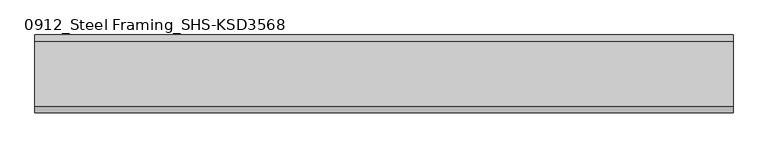
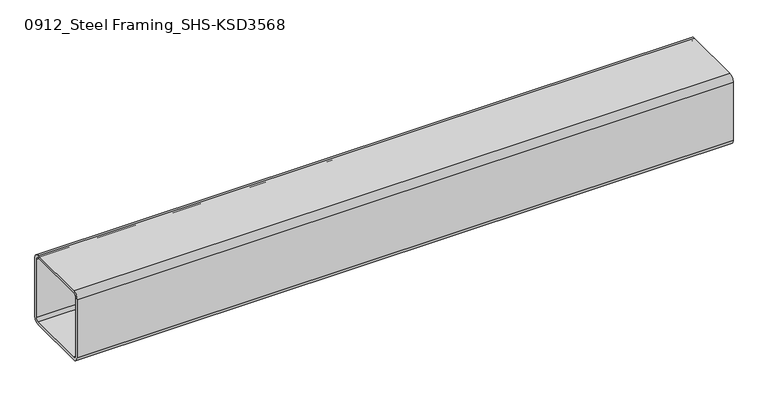
"""IFC4 building model written with IfcOpenShell, lengths in millimetres: beam geometry, 0912_Steel Framing_SHS-KSD3568 : H_SB_ASB_SHS-150x150x6."""

from ifc_helpers import new_model, si_unit, point, frame, frame_2d, origin, place, context, project, spatial, polyline, circle_curve, trimmed, segment, composite_curve, outline, extrude, source, transform, mapped, element, save


def beam_0912_steel_framing_shs_ksd3568_1769ed83(model_context):
    return source(origin(), model_context, "Body", "SweptSolid", [
        extrude(outline(composite_curve([segment(polyline([(75.0, 63.0), (75.0, -63.0)]), True, "CONTINUOUS"), segment(trimmed(circle_curve(frame_2d((63.0, -63.0)), 12.0), [point((75.0, -63.0))], [point((63.0, -75.0))], False, "CARTESIAN"), True, "CONTINUOUS"), segment(polyline([(63.0, -75.0), (-63.0, -75.0)]), True, "CONTINUOUS"), segment(trimmed(circle_curve(frame_2d((-63.0, -63.0)), 12.0), [point((-63.0, -75.0))], [point((-75.0, -63.0))], False, "CARTESIAN"), True, "CONTINUOUS"), segment(polyline([(-75.0, -63.0), (-75.0, 63.0)]), True, "CONTINUOUS"), segment(trimmed(circle_curve(frame_2d((-63.0, 63.0)), 12.0), [point((-75.0, 63.0))], [point((-63.0, 75.0))], False, "CARTESIAN"), True, "CONTINUOUS"), segment(polyline([(-63.0, 75.0), (63.0, 75.0)]), True, "CONTINUOUS"), segment(trimmed(circle_curve(frame_2d((63.0, 63.0)), 12.0), [point((63.0, 75.0))], [point((75.0, 63.0))], False, "CARTESIAN"), True, "CONTINUOUS")], self_intersect=False), holes=[composite_curve([segment(trimmed(circle_curve(frame_2d((-63.0, 63.0)), 6.0), [point((-63.0, 69.0))], [point((-69.0, 63.0))], True, "CARTESIAN"), True, "CONTINUOUS"), segment(polyline([(-69.0, 63.0), (-69.0, -63.0)]), True, "CONTINUOUS"), segment(trimmed(circle_curve(frame_2d((-63.0, -63.0)), 6.0), [point((-69.0, -63.0))], [point((-63.0, -69.0))], True, "CARTESIAN"), True, "CONTINUOUS"), segment(polyline([(-63.0, -69.0), (63.0, -69.0)]), True, "CONTINUOUS"), segment(trimmed(circle_curve(frame_2d((63.0, -63.0)), 6.0), [point((63.0, -69.0))], [point((69.0, -63.0))], True, "CARTESIAN"), True, "CONTINUOUS"), segment(polyline([(69.0, -63.0), (69.0, 63.0)]), True, "CONTINUOUS"), segment(trimmed(circle_curve(frame_2d((63.0, 63.0)), 6.0), [point((69.0, 63.0))], [point((63.0, 69.0))], True, "CARTESIAN"), True, "CONTINUOUS"), segment(polyline([(63.0, 69.0), (-63.0, 69.0)]), True, "CONTINUOUS")], self_intersect=False)]), frame((-674.1, 0.0, 0.0), z_axis=(1.0, 0.0, 0.0), x_axis=(0.0, 1.0, 0.0)), (0.0, 0.0, 1.0), 1348.2),
    ])


if __name__ == "__main__":
    model = new_model("IFC4")
    model_context = context("Model", 3, world=origin())
    ifc_project = project(units=[si_unit("LENGTHUNIT", "METRE", prefix="MILLI")], contexts=[model_context])
    site = spatial("IfcSite", under=ifc_project)
    building = spatial("IfcBuilding", under=site)
    placement = place(None, origin())
    beam_0912_steel_framing_shs_ksd3568_shape = beam_0912_steel_framing_shs_ksd3568_1769ed83(model_context)
    element("IfcBeam", 1, ObjectType="0912_Steel Framing_SHS-KSD3568 : H_SB_ASB_SHS-150x150x6", at=placement, inside=building, context=model_context, shape_type="MappedRepresentation", body=[
        mapped(beam_0912_steel_framing_shs_ksd3568_shape, transform((0.0, 0.0, 0.0), x_axis=(1.0, 0.0, 0.0), y_axis=(0.0, 1.0, 0.0), z_axis=(0.0, 0.0, 1.0))),
    ])
    save(model, "model.ifc")

# Revit data of these elements
# Type "0912_Steel Framing_SHS-KSD3568 : H_SB_ASB_SHS-150x150x6"
#   H_WM Code_1 = "S01AA002-00001 | Main Steel Structure Fabrication Work | Shelter/Building | Medium Steel - Standard (90KG/M>Weight≥30KG/M) | Material: (   )"
#   H_WM Code_2 = "S03AA028-00001 | Main Steel Structure Erection Work | Shelter/Building | Medium Steel (90KG/M>Weight≥30KG/M) | Material: (   )"
#   H_WM Code_3 = "S01AA010-00001 | Main Steel Structure Fabrication Work | Shelter/Building | Steel Painting/Coating | for Non-Fireproofed Steel Surface, Surface Preparation, Primer, Second & Final Coat | Material: (   )"
#   H_Q'ty Cal Type Tag = "SB-Q2"
#   Perimeter = 0.60 m²/m
#   Nominal Weight = 26.40 kgf/m
#   Length [instance default] = 1.0000 m
#   b = 0.1500 m
#   h = 0.1500 m
#   tr = 0.0120 m
#   t = 0.0060 m
#   A = 28.36 m²
#   Structural Material [instance default] = Steel, 45-345
# Element 1 (IfcBeam, "0912_Steel Framing_SHS-KSD3568 : H_SB_ASB_SHS-150x150x6")
#   Structural Material = none
# Materials
#   "Steel, 45-345": class "Metal", colour RGB 189 187 185, transparency 0, Description = "Steel 345 MPa", Cost = 0
